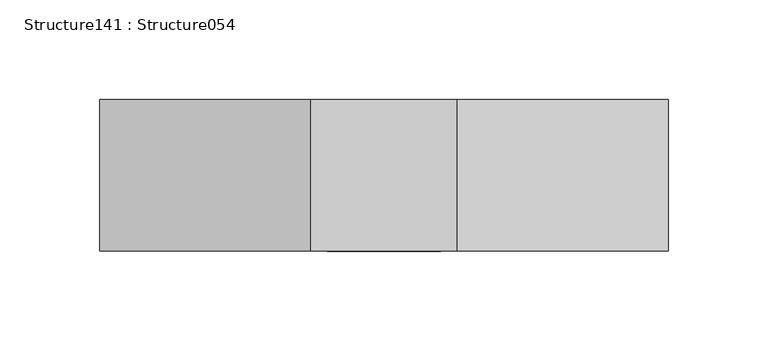
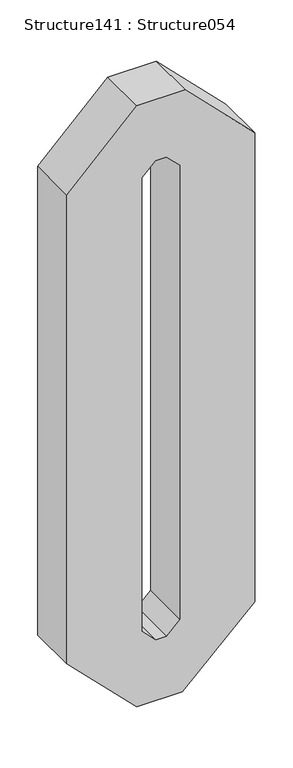
"""IFC4 building model written with IfcOpenShell, lengths in millimetres: proxy geometry, Structure141 : Structure054."""

from ifc_helpers import new_model, si_unit, frame, origin, place, context, project, spatial, polyline, outline, extrude, source, transform, mapped, element, save


def structure141_structure054_bf65ce99(model_context):
    return source(origin(), model_context, "Body", "SweptSolid", [
        extrude(outline(polyline([(4382.5453733, -49375.7559073), (3629.2077294, -49375.7559073), (3523.1417985, -49269.6899763), (3523.2149577, -49200.1951622), (3629.2065158, -49090.1917023), (4382.5456393, -49090.1904428), (4488.6115703, -49196.2563737), (4488.6115703, -49269.6899763), (4382.5453733, -49375.7559073)]), holes=[polyline([(3621.0476006, -49224.8139908), (3621.0482303, -49241.1285805), (3641.4463659, -49261.5266985), (4370.299463, -49261.5266985), (4390.697581, -49241.1285805), (4390.697581, -49224.813361), (4370.299463, -49204.415243), (3641.4461544, -49204.415243), (3621.0476006, -49224.8139908)])]), frame((0.0, 247945.1599557, 0.0), z_axis=(0.0, 1.0, 0.0), x_axis=(0.0, 0.0, 1.0)), (0.0, 0.0, 1.0), 76.2),
    ])


if __name__ == "__main__":
    model = new_model("IFC4")
    model_context = context("Model", 3, world=origin())
    ifc_project = project(units=[si_unit("LENGTHUNIT", "METRE", prefix="MILLI")], contexts=[model_context])
    site = spatial("IfcSite", under=ifc_project)
    building = spatial("IfcBuilding", under=site)
    placement = place(None, origin())
    structure141_structure054_shape = structure141_structure054_bf65ce99(model_context)
    element("IfcBuildingElementProxy", 1, Name="Structure141 : Structure054", ObjectType="Structure141 : Structure054", at=placement, inside=building, context=model_context, shape_type="MappedRepresentation", body=[
        mapped(structure141_structure054_shape, transform((0.0, 0.0, 0.0), x_axis=(1.0, 0.0, 0.0), y_axis=(0.0, 1.0, 0.0), z_axis=(0.0, 0.0, 1.0))),
    ])
    save(model, "model.ifc")

# Revit data of these elements
# Type "Structure141 : Structure054"
#   NameOverride = "Structure054"
# Element 1 (IfcBuildingElementProxy, "Structure141 : Structure054")
#   Materials on its faces: "BRUSHED ALUM. LETTERING"
# Materials
#   "BRUSHED ALUM. LETTERING": class "Unassigned", colour RGB 169 181 186, transparency 0, Cost = 0
